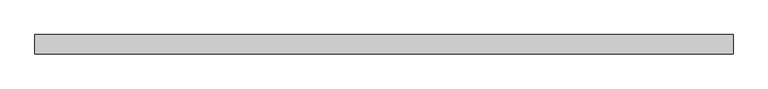
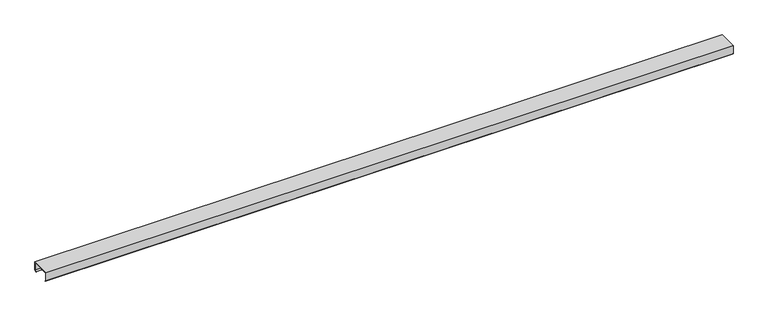
"""IFC4 building model written with IfcOpenShell, lengths in millimetres: proxy geometry, Generic Models 7:Generic Models 1:1:Generic Models 1:1 : Generic Models 7:Generic Models 1:337419:9 : Generic Models 7:Generic Models 1:1:Generic Models 1:1 : Generic Models 7:Generic Models 1:337419:306201."""

import ifcopenshell
import ifcopenshell.guid

model = None  # the IFC model being written
_history = None  # IfcOwnerHistory: only IFC2X3 demands one
_inside = {}  # id of a spatial element -> (the spatial element, [elements in it])
_under = {}  # id of a project, library or spatial element -> (it, [spatial elements below it])
_declared = {}  # id of a project -> (the project, [libraries it declares])
_typed = {}  # id of a type object -> (the type object, [elements of that type])
_made_of = {}  # id of a material, layer set ... -> (it, [elements and type objects made of it])


def new_model(schema):
    """Start an empty IFC model of exactly this schema.

    Asked for "IFC4X3", IfcOpenShell would pick the latest addendum, in which some entities
    have other attributes; the version numbers below select the first issue.
    IFC2X3 requires an IfcOwnerHistory on every rooted entity: one is made here for all.
    """
    global model, _history
    if schema == "IFC4X3":
        model = ifcopenshell.file(schema_version=(4, 3, 0, 0))
    else:
        model = ifcopenshell.file(schema=schema)
    _inside.clear()
    _under.clear()
    _declared.clear()
    _typed.clear()
    _made_of.clear()
    _history = None
    if model.schema == "IFC2X3":
        org = make("IfcOrganization", Name="unknown")
        user = make(
            "IfcPersonAndOrganization",
            ThePerson=make("IfcPerson", FamilyName="unknown"),
            TheOrganization=org,
        )
        app = make(
            "IfcApplication",
            ApplicationDeveloper=org,
            Version="unknown",
            ApplicationFullName="unknown",
            ApplicationIdentifier="unknown",
        )
        _history = make(
            "IfcOwnerHistory",
            OwningUser=user,
            OwningApplication=app,
            ChangeAction="ADDED",
            CreationDate=0,
        )
    return model


def make(cls, **values):
    """One entity of the class cls with the attributes given. An attribute that is None is left unset."""
    return model.create_entity(
        cls, **{name: value for name, value in values.items() if value is not None}
    )


def rooted(cls, **values):
    """An entity with a GlobalId (a new one), such as an element, a storey or a relation."""
    return make(cls, GlobalId=ifcopenshell.guid.new(), OwnerHistory=_history, **values)


def si_unit(unit_type, name, prefix=None):
    """IfcSIUnit, for example si_unit("LENGTHUNIT", "METRE", prefix="MILLI")."""
    return make("IfcSIUnit", UnitType=unit_type, Prefix=prefix, Name=name)


def assignment(units):
    """IfcUnitAssignment: the units of a project."""
    return None if units is None else make("IfcUnitAssignment", Units=units)


def point(xyz):
    """IfcCartesianPoint."""
    return None if xyz is None else make("IfcCartesianPoint", Coordinates=xyz)


def direction(xyz):
    """IfcDirection."""
    return None if xyz is None else make("IfcDirection", DirectionRatios=xyz)


def frame(location, z_axis=None, x_axis=None):
    """IfcAxis2Placement3D, a coordinate frame: its origin and axes. An axis left out is left unset."""
    return make(
        "IfcAxis2Placement3D",
        Location=point(location),
        Axis=direction(z_axis),
        RefDirection=direction(x_axis),
    )


def origin():
    """The frame at (0, 0, 0) with its axes left unset."""
    return frame((0.0, 0.0, 0.0))


def place(relative_to, where):
    """IfcLocalPlacement: puts the frame where relative to a parent placement (None: the world)."""
    return make(
        "IfcLocalPlacement", PlacementRelTo=relative_to, RelativePlacement=where
    )


def context(
    kind, dimensions, precision=None, world=None, true_north=None, identifier=None
):
    """IfcGeometricRepresentationContext, for example the 3D "Model" context."""
    return make(
        "IfcGeometricRepresentationContext",
        ContextIdentifier=identifier,
        ContextType=kind,
        CoordinateSpaceDimension=dimensions,
        Precision=precision,
        WorldCoordinateSystem=world,
        TrueNorth=true_north,
    )


def project(units=None, contexts=None):
    """IfcProject with its units and contexts."""
    return rooted(
        "IfcProject",
        Name="project",
        RepresentationContexts=contexts,
        UnitsInContext=assignment(units),
    )


def spatial(cls, under=None, at=None, **own):
    """A site, building, storey or space (cls), placed at a placement, below another one or the project."""
    s = rooted(cls, ObjectPlacement=at, **own)
    if under is not None:
        _under.setdefault(under.id(), (under, []))[1].append(s)
    return s


def polyline(points):
    """IfcPolyline through the points."""
    return make("IfcPolyline", Points=[point(p) for p in points])


def outline(outer, holes=None, kind="AREA"):
    """IfcArbitraryClosedProfileDef: a profile drawn as a closed curve; with holes, ...WithVoids."""
    if holes is None:
        return make("IfcArbitraryClosedProfileDef", ProfileType=kind, OuterCurve=outer)
    return make(
        "IfcArbitraryProfileDefWithVoids",
        ProfileType=kind,
        OuterCurve=outer,
        InnerCurves=holes,
    )


def extrude(swept, where, along, depth):
    """IfcExtrudedAreaSolid: the profile swept, set in the frame where, extruded along a direction by depth."""
    return make(
        "IfcExtrudedAreaSolid",
        SweptArea=swept,
        Position=where,
        ExtrudedDirection=direction(along),
        Depth=depth,
    )


def shape(context_of_items, identifier, shape_type, items):
    """IfcShapeRepresentation: the items that make up one representation, for example the "Body"."""
    return make(
        "IfcShapeRepresentation",
        ContextOfItems=context_of_items,
        RepresentationIdentifier=identifier,
        RepresentationType=shape_type,
        Items=items,
    )


def source(mapping_origin, context_of_items, identifier, shape_type, items):
    """IfcRepresentationMap: a shape defined once, which mapped items show again and again."""
    return make(
        "IfcRepresentationMap",
        MappingOrigin=mapping_origin,
        MappedRepresentation=shape(context_of_items, identifier, shape_type, items),
    )


def transform(
    local_origin,
    x_axis=None,
    y_axis=None,
    z_axis=None,
    scale=None,
    scale2=None,
    scale3=None,
    uniform=True,
):
    """IfcCartesianTransformationOperator3D, or its non-uniform kind. x_axis, y_axis, z_axis: its Axis1, 2, 3."""
    if uniform:
        return make(
            "IfcCartesianTransformationOperator3D",
            Axis1=direction(x_axis),
            Axis2=direction(y_axis),
            LocalOrigin=point(local_origin),
            Scale=scale,
            Axis3=direction(z_axis),
        )
    return make(
        "IfcCartesianTransformationOperator3DnonUniform",
        Axis1=direction(x_axis),
        Axis2=direction(y_axis),
        LocalOrigin=point(local_origin),
        Scale=scale,
        Axis3=direction(z_axis),
        Scale2=scale2,
        Scale3=scale3,
    )


def mapped(mapping_source, mapping_target):
    """IfcMappedItem: shows the shape of a source again, moved by a transform."""
    return make(
        "IfcMappedItem", MappingSource=mapping_source, MappingTarget=mapping_target
    )


def made_of(thing, what):
    """Note that an element or type object is made of a material, layer set ...; save() writes the relation."""
    if what is not None:
        _made_of.setdefault(what.id(), (what, []))[1].append(thing)
    return thing


def element(
    cls,
    number,
    at=None,
    inside=None,
    cuts=None,
    type_object=None,
    material=None,
    context=None,
    identifier="Body",
    shape_type=None,
    held_by="IfcProductDefinitionShape",
    body=None,
    shapes=None,
    **own,
):
    """One element of the class cls, such as IfcWall. Its Tag is "e" and its number.

    at: its placement. inside: the storey or other place that contains it. cuts: it is an
    opening in that element (IfcRelVoidsElement). A single representation is given by context,
    identifier, shape_type and body (its items); several are given by shapes. held_by: the class
    of the entity that holds the representations. save() writes the other relations.
    """
    e = rooted(cls, Tag="e%d" % number, ObjectPlacement=at, **own)
    if body is not None:
        shapes = [shape(context, identifier, shape_type, body)]
    if shapes is not None:
        e.Representation = make(held_by, Representations=shapes)
    if inside is not None:
        _inside.setdefault(inside.id(), (inside, []))[1].append(e)
    if cuts is not None:
        rooted(
            "IfcRelVoidsElement", RelatingBuildingElement=cuts, RelatedOpeningElement=e
        )
    if type_object is not None:
        _typed.setdefault(type_object.id(), (type_object, []))[1].append(e)
    return made_of(e, material)


def aggregate(whole, parts):
    """IfcRelAggregates: a whole, such as a stair, and the parts it consists of."""
    return rooted("IfcRelAggregates", RelatingObject=whole, RelatedObjects=parts)


def save(model, path):
    """Write the relations noted so far, then the file.

    IfcRelAggregates (storeys below a building ...), IfcRelContainedInSpatialStructure (elements
    in a storey), IfcRelDefinesByType, IfcRelAssociatesMaterial and IfcRelDeclares: one each for
    every whole, place, type object, material and project.
    """
    for whole, parts in _under.values():
        aggregate(whole, parts)
    for where, things in _inside.values():
        rooted(
            "IfcRelContainedInSpatialStructure",
            RelatedElements=things,
            RelatingStructure=where,
        )
    for kind, things in _typed.values():
        rooted("IfcRelDefinesByType", RelatedObjects=things, RelatingType=kind)
    for what, things in _made_of.values():
        rooted("IfcRelAssociatesMaterial", RelatedObjects=things, RelatingMaterial=what)
    for by, libraries in _declared.values():
        rooted("IfcRelDeclares", RelatingContext=by, RelatedDefinitions=libraries)
    model.write(path)


def generic_models_0c1aad58(model_context):
    return source(origin(), model_context, "Body", "SweptSolid", [
        extrude(outline(polyline([(-579000.6913841, 6128.940625), (-578797.4913841, 6128.940625), (-578797.4913841, 6040.040625), (-578812.0845307, 6027.7955211), (-578813.8702751, 6029.9236883), (-578800.2695091, 6041.336086), (-578800.2695091, 6126.1625), (-578997.9132591, 6126.1625), (-578997.9132591, 6041.336086), (-578984.3124931, 6029.9236883), (-578986.0982375, 6027.7955211), (-579000.6913841, 6040.040625), (-579000.6913841, 6128.940625)])), frame((565582.1867239, 0.0, 0.0), z_axis=(1.0, 0.0, 0.0), x_axis=(0.0, 1.0, 0.0)), (0.0, 0.0, 1.0), 7315.2),
    ])


if __name__ == "__main__":
    model = new_model("IFC4")
    model_context = context("Model", 3, world=origin())
    ifc_project = project(units=[si_unit("LENGTHUNIT", "METRE", prefix="MILLI")], contexts=[model_context])
    site = spatial("IfcSite", under=ifc_project)
    building = spatial("IfcBuilding", under=site)
    placement = place(None, origin())
    generic_models_shape = generic_models_0c1aad58(model_context)
    element("IfcBuildingElementProxy", 1, Name="Generic Models 7:Generic Models 1:1:Generic Models 1:1 : Generic Models 7:Generic Models 1:337419:9 : Generic Models 7:Generic Models 1:1:Generic Models 1:1 : Generic Models 7:Generic Models 1:337419:306201", ObjectType="Generic Models 7:Generic Models 1:1:Generic Models 1:1 : Generic Models 7:Generic Models 1:337419:9 : Generic Models 7:Generic Models 1:1:Generic Models 1:1 : Generic Models 7:Generic Models 1:337419:306201", at=placement, inside=building, context=model_context, shape_type="MappedRepresentation", body=[
        mapped(generic_models_shape, transform((0.0, 0.0, 0.0), x_axis=(1.0, 0.0, 0.0), y_axis=(0.0, 1.0, 0.0), z_axis=(0.0, 0.0, 1.0))),
    ])
    save(model, "model.ifc")

# Revit data of these elements
# Type "Generic Models 7:Generic Models 1:1:Generic Models 1:1 : Generic Models 7:Generic Models 1:337419:9 : Generic Models 7:Generic Models 1:1:Generic Models 1:1 : Generic Models 7:Generic Models 1:337419:306201"
#   NameOverride = "Generic Models 7:Generic Models 1:1:Generic Models 1:1 : Generic Models 7:Generic Models 1:337419:306201"
#   ObjectTypeOverride = "Generic Models 1:1 : Generic Models 7:Generic Models 1:337419"
#   Reference = "Generic Models 1"
#   Tag = "306201"
# Element 1 (IfcBuildingElementProxy, "Generic Models 7:Generic Models 1:1:Generic Models 1:1 : Generic Models 7:Generic Models 1:337419:9 : Generic Models 7:Generic Models 1:1:Generic Models 1:1 : Generic Models 7:Generic Models 1:337419:306201")
#   Materials on its faces: "CEE' SECTION (8.0x3.5C - SEE STRUCT. DWGS)"
# Materials
#   "CEE' SECTION (8.0x3.5C - SEE STRUCT. DWGS)": class "Unassigned", colour RGB 210 209 208, transparency 0, Keynote = "M05121300.02", Cost = 0
